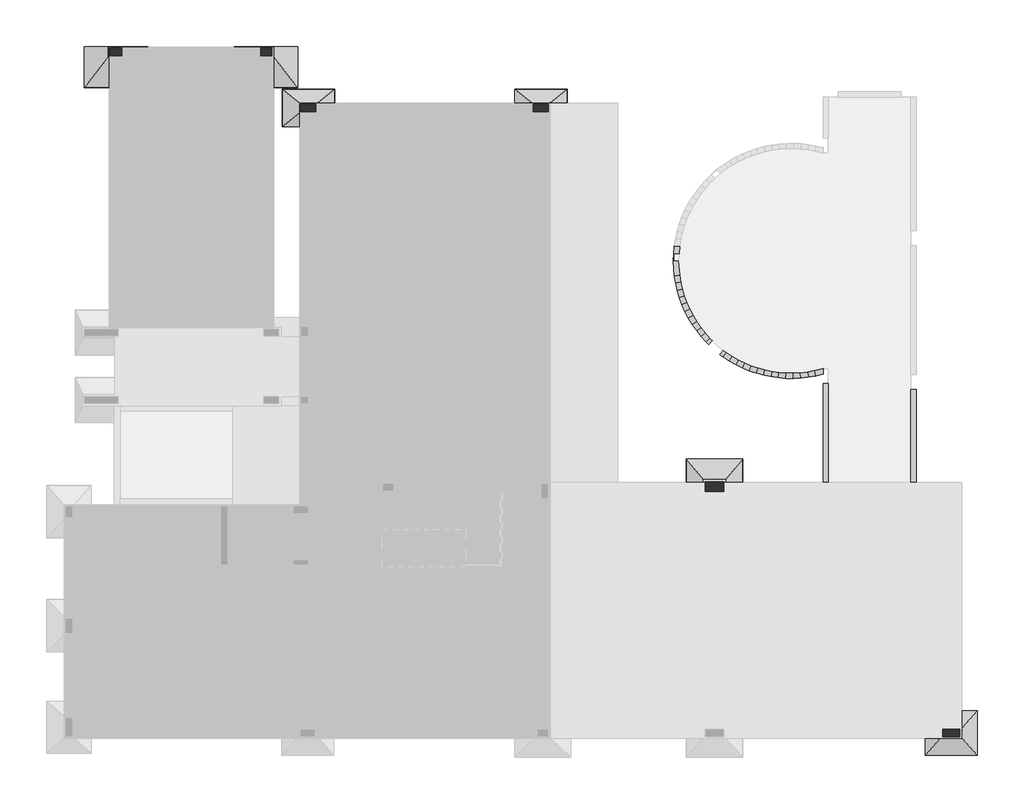
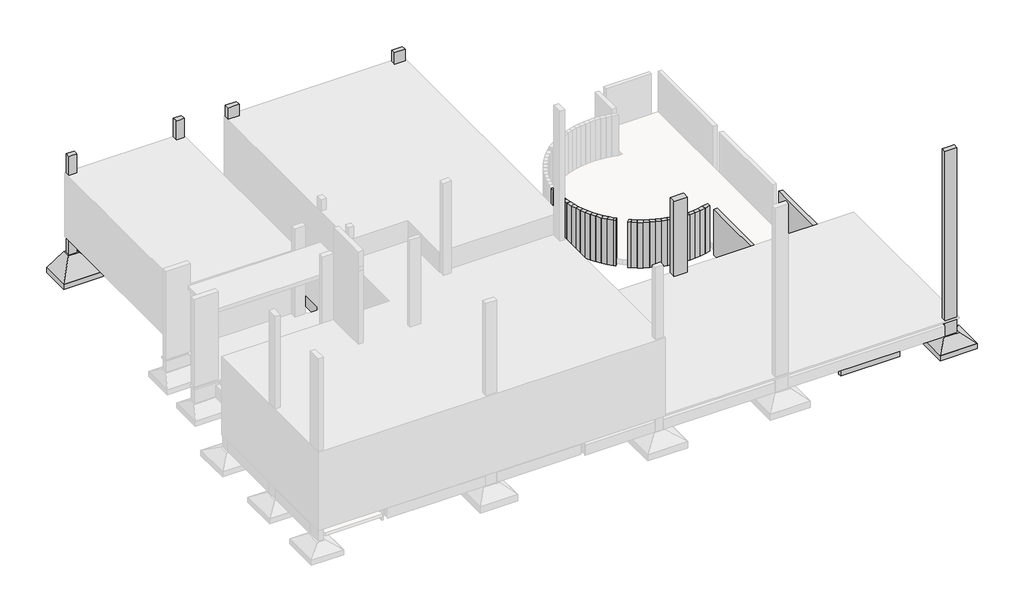
# One storey, part 3 of 4: 35 beams, 7 fasteners, 6 columns.
# Revit data of these elements (continued)
# Element 42 (IfcFastener, "TQS - Sapata : S1") (continued)
#   Casos de vento manual = ""
#   Tipo = "Sapata"
#   Dimensoes = "110.0,170.0"
#   Estacas = ""
#   Calice = ""
#   Rugosidade = ""
#   Alcas = ""
#   Furos = ""
#   Pino = ""
#   Distribuicao = ""
#   Solidarizado = ""
#   Solidarizar na montagem = ""
#   Unir com o próximo = ""
#   Grupo pre moldado = ""
#   Verificado = ""
#   Concreto C = ""
#   Taxa de armadura (kgf/m³) = 0
#   Carga (tf/m²) = 0
#   Carga (tf/m) = 0
#   Carga (tf) = 0
#   Altura = 0.00 m
#   Rebaixo = 0.00 m
#   Pilar ficticio = 0.00 m
#   Topo = -0.10 m
#   Altura total = 0.60 m
#   Rodape = 0.00 m
#   Diametro = 0.00 m
#   Altura dentro do bloco = 0.00 m
#   Entre eixos = 0.00 m
#   Paredes = 0.00 m
#   Caimento = 0.00 m
#   Largura = 0.00 m
#   Distancia a face = 0.00 m
#   Distancia ao eixo = 0.00 m
#   Resultado de Ensaios fck (MPa) = 0
#   Unique TQS ID = -1407
#   Principal = yes
#   Phase Created = CC_AP/ESTR
#   Materials on its faces: "Concreto - Concreto concretado no local"
# Element 43 (IfcFastener, "TQS - Sapata : S12")
#   Uso = "ESTRUTURA"
#   Titulo = "S12"
#   Chave = "-1436"
#   Tipo Elemento = "Fundação"
#   SHA1 = "A28B53AB49304EFCBF9C768E884AA5FFCB5BBDAA"
#   Revisão = ""
#   Tipo de carga = ""
#   Divisor de flexao = ""
#   Secao = ""
#   Configuracao = ""
#   Angulo (graus) = ""
#   Detalhamento = ""
#   Casos de vento manual = ""
#   Tipo = "Sapata"
#   Dimensoes = "150.0,150.0"
#   Estacas = ""
#   Calice = ""
#   Rugosidade = ""
#   Alcas = ""
#   Furos = ""
#   Pino = ""
#   Distribuicao = ""
#   Solidarizado = ""
#   Solidarizar na montagem = ""
#   Unir com o próximo = ""
#   Grupo pre moldado = ""
#   Verificado = ""
#   Concreto C = ""
#   Taxa de armadura (kgf/m³) = 0
#   Carga (tf/m²) = 0
#   Carga (tf/m) = 0
#   Carga (tf) = 0
#   Altura = 0.00 m
#   Rebaixo = 0.00 m
#   Pilar ficticio = 0.00 m
#   Topo = -0.10 m
#   Altura total = 0.60 m
#   Rodape = 0.00 m
#   Diametro = 0.00 m
#   Altura dentro do bloco = 0.00 m
#   Entre eixos = 0.00 m
#   Paredes = 0.00 m
#   Caimento = 0.00 m
#   Largura = 0.00 m
#   Distancia a face = 0.00 m
#   Distancia ao eixo = 0.00 m
#   Resultado de Ensaios fck (MPa) = 0
#   Unique TQS ID = -1436
#   Principal = yes
#   Phase Created = CC_AP/ESTR
#   Materials on its faces: "Concreto - Concreto concretado no local"
# Element 44 (IfcFastener, "TQS - Sapata : S13")
#   Uso = "ESTRUTURA"
#   Titulo = "S13"
#   Chave = "-1457"
#   Tipo Elemento = "Fundação"
#   SHA1 = "BF7891B0F83325896F70E9D7259C0573D0C4C40D"
#   Revisão = ""
#   Tipo de carga = ""
#   Divisor de flexao = ""
#   Secao = ""
#   Configuracao = ""
#   Angulo (graus) = ""
#   Detalhamento = ""
#   Casos de vento manual = ""
#   Tipo = "Sapata"
#   Dimensoes = "150.0,150.0"
#   Estacas = ""
#   Calice = ""
#   Rugosidade = ""
#   Alcas = ""
#   Furos = ""
#   Pino = ""
#   Distribuicao = ""
#   Solidarizado = ""
#   Solidarizar na montagem = ""
#   Unir com o próximo = ""
#   Grupo pre moldado = ""
#   Verificado = ""
#   Concreto C = ""
#   Taxa de armadura (kgf/m³) = 0
#   Carga (tf/m²) = 0
#   Carga (tf/m) = 0
#   Carga (tf) = 0
#   Altura = 0.00 m
#   Rebaixo = 0.00 m
#   Pilar ficticio = 0.00 m
#   Topo = -0.10 m
#   Altura total = 0.50 m
#   Rodape = 0.00 m
#   Diametro = 0.00 m
#   Altura dentro do bloco = 0.00 m
#   Entre eixos = 0.00 m
#   Paredes = 0.00 m
#   Caimento = 0.00 m
#   Largura = 0.00 m
#   Distancia a face = 0.00 m
#   Distancia ao eixo = 0.00 m
#   Resultado de Ensaios fck (MPa) = 0
#   Unique TQS ID = -1457
#   Principal = yes
#   Phase Created = CC_AP/ESTR
#   Materials on its faces: "Concreto - Concreto concretado no local"
# Element 45 (IfcFastener, "TQS - Sapata : S2")
#   Uso = "ESTRUTURA"
#   Titulo = "S2"
#   Chave = "-1408"
#   Tipo Elemento = "Fundação"
#   SHA1 = "2282C10FF7FA64FC48FCFA0318D48FBC3A2ACDAC"
#   Revisão = ""
#   Tipo de carga = ""
#   Divisor de flexao = ""
#   Secao = ""
#   Configuracao = ""
#   Angulo (graus) = ""
#   Detalhamento = ""
#   Casos de vento manual = ""
#   Tipo = "Sapata"
#   Dimensoes = "110.0,170.0"
#   Estacas = ""
#   Calice = ""
#   Rugosidade = ""
#   Alcas = ""
#   Furos = ""
#   Pino = ""
#   Distribuicao = ""
#   Solidarizado = ""
#   Solidarizar na montagem = ""
#   Unir com o próximo = ""
#   Grupo pre moldado = ""
#   Verificado = ""
#   Concreto C = ""
#   Taxa de armadura (kgf/m³) = 0
#   Carga (tf/m²) = 0
#   Carga (tf/m) = 0
#   Carga (tf) = 0
#   Altura = 0.00 m
#   Rebaixo = 0.00 m
#   Pilar ficticio = 0.00 m
#   Topo = -0.10 m
#   Altura total = 0.60 m
#   Rodape = 0.00 m
#   Diametro = 0.00 m
#   Altura dentro do bloco = 0.00 m
#   Entre eixos = 0.00 m
#   Paredes = 0.00 m
#   Caimento = 0.00 m
#   Largura = 0.00 m
#   Distancia a face = 0.00 m
#   Distancia ao eixo = 0.00 m
#   Resultado de Ensaios fck (MPa) = 0
#   Unique TQS ID = -1408
#   Principal = yes
#   Phase Created = CC_AP/ESTR
#   Materials on its faces: "Concreto - Concreto concretado no local"
# Element 46 (IfcFastener, "TQS - Sapata : S24")
#   Uso = "ESTRUTURA"
#   Titulo = "S24"
#   Chave = "-1461"
#   Tipo Elemento = "Fundação"
#   SHA1 = "7859DB63F09D5F0F67BBBF72A3CA603880B25958"
#   Revisão = ""
#   Tipo de carga = ""
#   Divisor de flexao = ""
#   Secao = ""
#   Configuracao = ""
#   Angulo (graus) = ""
#   Detalhamento = ""
#   Casos de vento manual = ""
#   Tipo = "Sapata"
#   Dimensoes = "120.0,140.0"
#   Estacas = ""
#   Calice = ""
#   Rugosidade = ""
#   Alcas = ""
#   Furos = ""
#   Pino = ""
#   Distribuicao = ""
#   Solidarizado = ""
#   Solidarizar na montagem = ""
#   Unir com o próximo = ""
#   Grupo pre moldado = ""
#   Verificado = ""
#   Concreto C = ""
#   Taxa de armadura (kgf/m³) = 0
#   Carga (tf/m²) = 0
#   Carga (tf/m) = 0
#   Carga (tf) = 0
#   Altura = 0.00 m
#   Rebaixo = 0.00 m
#   Pilar ficticio = 0.00 m
#   Topo = -0.06 m
#   Altura total = 0.50 m
#   Rodape = 0.00 m
#   Diametro = 0.00 m
#   Altura dentro do bloco = 0.00 m
#   Entre eixos = 0.00 m
#   Paredes = 0.00 m
#   Caimento = 0.00 m
#   Largura = 0.00 m
#   Distancia a face = 0.00 m
#   Distancia ao eixo = 0.00 m
#   Resultado de Ensaios fck (MPa) = 0
#   Unique TQS ID = -1461
#   Principal = yes
#   Phase Created = CC_AP/ESTR
#   Materials on its faces: "Concreto - Concreto concretado no local"
# Element 47 (IfcFastener, "TQS - Sapata : S3")
#   Uso = "ESTRUTURA"
#   Titulo = "S3"
#   Chave = "-1405"
#   Tipo Elemento = "Fundação"
#   SHA1 = "E7F86A4529557F0178A31412CAAF120C6199F7FB"
#   Revisão = ""
#   Tipo de carga = ""
#   Divisor de flexao = ""
#   Secao = ""
#   Configuracao = ""
#   Angulo (graus) = ""
#   Detalhamento = ""
#   Casos de vento manual = ""
#   Tipo = "Sapata"
#   Dimensoes = "100.0,140.0"
#   Estacas = ""
#   Calice = ""
#   Rugosidade = ""
#   Alcas = ""
#   Furos = ""
#   Pino = ""
#   Distribuicao = ""
#   Solidarizado = ""
#   Solidarizar na montagem = ""
#   Unir com o próximo = ""
#   Grupo pre moldado = ""
#   Verificado = ""
#   Concreto C = ""
#   Taxa de armadura (kgf/m³) = 0
#   Carga (tf/m²) = 0
#   Carga (tf/m) = 0
#   Carga (tf) = 0
#   Altura = 0.00 m
#   Rebaixo = 0.00 m
#   Pilar ficticio = 0.00 m
#   Topo = 0.00 m
#   Altura total = 0.50 m
#   Rodape = 0.00 m
#   Diametro = 0.00 m
#   Altura dentro do bloco = 0.00 m
#   Entre eixos = 0.00 m
#   Paredes = 0.00 m
#   Caimento = 0.00 m
#   Largura = 0.00 m
#   Distancia a face = 0.00 m
#   Distancia ao eixo = 0.00 m
#   Resultado de Ensaios fck (MPa) = 0
#   Unique TQS ID = -1405
#   Principal = yes
#   Phase Created = CC_AP/ESTR
#   Materials on its faces: "Concreto - Concreto concretado no local"
# Element 48 (IfcFastener, "TQS - Sapata : S4")
#   Uso = "ESTRUTURA"
#   Titulo = "S4"
#   Chave = "-1406"
#   Tipo Elemento = "Fundação"
#   SHA1 = "1CBAC234F592DF4B85828C708D4D8DF50E3056D8"
#   Revisão = ""
#   Tipo de carga = ""
#   Divisor de flexao = ""
#   Secao = ""
#   Configuracao = ""
#   Angulo (graus) = ""
#   Detalhamento = ""
#   Casos de vento manual = ""
#   Tipo = "Sapata"
#   Dimensoes = "100.0,140.0"
#   Estacas = ""
#   Calice = ""
#   Rugosidade = ""
#   Alcas = ""
#   Furos = ""
#   Pino = ""
#   Distribuicao = ""
#   Solidarizado = ""
#   Solidarizar na montagem = ""
#   Unir com o próximo = ""
#   Grupo pre moldado = ""
#   Verificado = ""
#   Concreto C = ""
#   Taxa de armadura (kgf/m³) = 0
#   Carga (tf/m²) = 0
#   Carga (tf/m) = 0
#   Carga (tf) = 0
#   Altura = 0.00 m
#   Rebaixo = 0.00 m
#   Pilar ficticio = 0.00 m
#   Topo = 0.00 m
#   Altura total = 0.50 m
#   Rodape = 0.00 m
#   Diametro = 0.00 m
#   Altura dentro do bloco = 0.00 m
#   Entre eixos = 0.00 m
#   Paredes = 0.00 m
#   Caimento = 0.00 m
#   Largura = 0.00 m
#   Distancia a face = 0.00 m
#   Distancia ao eixo = 0.00 m
#   Resultado de Ensaios fck (MPa) = 0
#   Unique TQS ID = -1406
#   Principal = yes
#   Phase Created = CC_AP/ESTR
#   Materials on its faces: "Concreto - Concreto concretado no local"
# Materials
#   "Concrete - Cast-in-Place Concrete": class "Unassigned", colour RGB 192 192 192, transparency 0
#   "Concreto - Concreto concretado no local": class "Concreto", colour RGB 192 192 192, transparency 0
